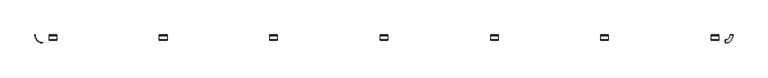
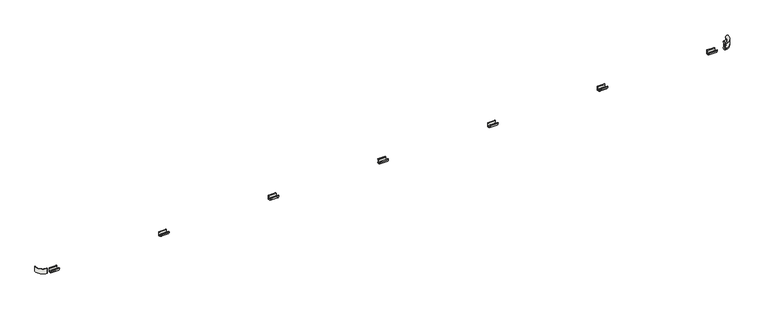
"""IFC4 building model written with IfcOpenShell, lengths in millimetres: covering geometry, Construction_Railing_SPM_Starline-Anodisee-Decowood : Decowood."""

from ifc_helpers import new_model, si_unit, point, frame, frame_2d, origin, place, context, project, spatial, polyline, circle_curve, ellipse_curve, trimmed, segment, composite_curve, outline, extrude, source, transform, mapped, element, save
from ifc_brep_helpers import plane_surface, cylinder_surface, revolved_surface, advanced_brep


def covering_9951a4d6(model_context):
    return source(origin(), model_context, "Body", "SolidModel", [
        advanced_brep(
        [(5562.5, 0.0, 711.0388007), (5562.5, -1.6924902, 711.0388007), (5562.5, -1.6924902, 680.0573863), (5562.5, 0.0, 680.0573863), (5562.5, 0.0, 675.0589555), (5562.5, -4.6960308, 675.0589555), (5562.5, -53.704315, 715.3021276), (5562.5, -51.003274, 720.0337391), (5562.5, -48.3728597, 720.0337391), (5562.5, -11.4596372, 681.5800945), (5562.5, -5.6906152, 686.5206011), (5562.5, -5.6906152, 712.273279), (5562.5, -1.927393, 716.0365012), (5562.5, 0.0, 716.0365012), (5637.5, 0.0, 711.0388007), (5637.5, 0.0, 716.0365012), (5637.5, -1.927393, 716.0365012), (5637.5, -5.6906152, 712.273279), (5637.5, -5.6906152, 686.5206011), (5637.5, -11.4596372, 681.5800945), (5637.5, -48.3728597, 720.0337391), (5637.5, -51.003274, 720.0337391), (5637.5, -53.704315, 715.3021276), (5637.5, -4.6960308, 675.059214), (5637.5, 0.0, 675.0589555), (5637.5, 0.0, 680.0573863), (5637.5, -1.6924902, 680.0573863), (5637.5, -1.6924902, 711.0388007)],
        [
            (0, 1),
            (1, 2),
            (2, 3),
            (3, 4),
            (4, 5),
            (5, 6, circle_curve(frame((5562.5, -4.6960308, 725.0220975), z_axis=(-1.0, 0.0, 0.0), x_axis=(0.0, 0.0, 1.0)), 49.9628835)),
            (6, 7, circle_curve(frame((5562.5, -65.1640589, 724.9806745), z_axis=(1.0, 0.0, 0.0), x_axis=(0.0, 0.0, 1.0)), 15.0)),
            (7, 8),
            (8, 9, circle_curve(frame((5562.5, -4.6988472, 725.0141293), z_axis=(1.0, 0.0, 0.0), x_axis=(0.0, 0.0, 1.0)), 43.957066)),
            (9, 10, circle_curve(frame((5562.5, -10.6906152, 686.5206011), z_axis=(1.0, 0.0, 0.0), x_axis=(0.0, 0.0, 1.0)), 5.0)),
            (10, 11),
            (11, 12, circle_curve(frame((5562.5, -1.927393, 712.273279), z_axis=(-1.0, 0.0, 0.0), x_axis=(0.0, 0.0, 1.0)), 3.7632222)),
            (12, 13),
            (13, 0),
            (14, 15),
            (15, 16),
            (16, 17, circle_curve(frame((5637.5, -1.927393, 712.273279), z_axis=(1.0, 0.0, 0.0), x_axis=(0.0, 0.0, 1.0)), 3.7632222)),
            (17, 18),
            (18, 19, circle_curve(frame((5637.5, -10.6906152, 686.5206011), z_axis=(-1.0, 0.0, 0.0), x_axis=(0.0, 0.0, 1.0)), 5.0)),
            (19, 20, circle_curve(frame((5637.5, -4.6988472, 725.0141293), z_axis=(-1.0, 0.0, 0.0), x_axis=(0.0, 0.0, 1.0)), 43.957066)),
            (20, 21),
            (21, 22, circle_curve(frame((5637.5, -65.1640589, 724.9806745), z_axis=(-1.0, 0.0, 0.0), x_axis=(0.0, 0.0, 1.0)), 15.0)),
            (22, 23, circle_curve(frame((5637.5, -4.6960308, 725.0220975), z_axis=(1.0, 0.0, 0.0), x_axis=(0.0, 0.0, 1.0)), 49.9628835)),
            (23, 24),
            (24, 25),
            (25, 26),
            (26, 27),
            (27, 14),
            (0, 14),
            (27, 1),
            (26, 2),
            (25, 3),
            (24, 4),
            (23, 5),
            (22, 6),
            (21, 7),
            (20, 8),
            (19, 9),
            (18, 10),
            (17, 11),
            (16, 12),
            (15, 13),
        ],
        [
            plane_surface(frame((5562.5, -1.6924902, 711.0388007), z_axis=(-1.0, 0.0, 0.0), x_axis=(0.0, -1.0, 0.0))),
            plane_surface(frame((5637.5, -1.6924902, 711.0388007), z_axis=(1.0, 0.0, 0.0), x_axis=(0.0, 1.0, 0.0))),
            plane_surface(frame((5562.5, 0.0, 711.0388007), z_axis=(0.0, 0.0, -1.0), x_axis=(1.0, 0.0, 0.0))),
            plane_surface(frame((5562.5, -1.6924902, 711.0388007), z_axis=(0.0, 1.0, 0.0), x_axis=(1.0, 0.0, 0.0))),
            plane_surface(frame((5562.5, -1.6924902, 680.0573863), z_axis=(0.0, 0.0, 1.0), x_axis=(1.0, 0.0, 0.0))),
            plane_surface(frame((5562.5, 0.0, 680.0573863), z_axis=(0.0, 1.0, 0.0), x_axis=(1.0, 0.0, 0.0))),
            plane_surface(frame((5562.5, 0.0, 675.0589555), z_axis=(0.0, 0.0, -1.0), x_axis=(1.0, 0.0, 0.0))),
            cylinder_surface(frame((5637.5, -4.6960308, 725.0220975), z_axis=(-1.0, 0.0, 0.0), x_axis=(0.0, 0.0, 1.0)), 49.9628835),
            revolved_surface(polyline([(5637.5, -65.1640589, 739.9806745), (5562.5, -65.1640589, 739.9806745)]), (5637.5, -65.1640589, 724.9806745), (1.0, 0.0, 0.0)),
            plane_surface(frame((5562.5, -51.003274, 720.0337391), z_axis=(0.0, 0.0, 1.0), x_axis=(1.0, 0.0, 0.0))),
            revolved_surface(polyline([(5637.5, -4.6988472, 768.9711953000001), (5562.5, -4.6988472, 768.9711953000001)]), (5637.5, -4.6988472, 725.0141293), (1.0, 0.0, 0.0)),
            revolved_surface(polyline([(5637.5, -10.6906152, 691.5206011), (5562.5, -10.6906152, 691.5206011)]), (5637.5, -10.6906152, 686.5206011), (1.0, 0.0, 0.0)),
            plane_surface(frame((5562.5, -5.6906152, 686.5206011), z_axis=(0.0, -1.0, 0.0), x_axis=(1.0, 0.0, 0.0))),
            cylinder_surface(frame((5637.5, -1.927393, 712.273279), z_axis=(-1.0, 0.0, 0.0), x_axis=(0.0, 0.0, 1.0)), 3.7632222),
            plane_surface(frame((5562.5, -1.927393, 716.0365012), z_axis=(0.0, 0.0, 1.0), x_axis=(1.0, 0.0, 0.0))),
            plane_surface(frame((5562.5, 0.0, 716.0365012), z_axis=(0.0, 1.0, 0.0), x_axis=(1.0, 0.0, 0.0))),
        ],
        [
            (0, [[1, 2, 3, 4, 5, 6, 7, 8, 9, 10, 11, 12, 13, 14]]),
            (1, [[15, 16, 17, 18, 19, 20, 21, 22, 23, 24, 25, 26, 27, 28]]),
            (2, [[-1, 29, -28, 30]]),
            (3, [[-2, -30, -27, 31]]),
            (4, [[-3, -31, -26, 32]]),
            (5, [[-4, -32, -25, 33]]),
            (6, [[-5, -33, -24, 34]]),
            (7, [[-6, -34, -23, 35]]),
            (8, [[-7, -35, -22, 36]]),
            (9, [[-8, -36, -21, 37]]),
            (10, [[-9, -37, -20, 38]]),
            (11, [[-10, -38, -19, 39]]),
            (12, [[-11, -39, -18, 40]]),
            (13, [[-12, -40, -17, 41]]),
            (14, [[-13, -41, -16, 42]]),
            (15, [[-14, -42, -15, -29]]),
        ],
    ),
        advanced_brep(
        [(4462.5, 0.0, 711.0388007), (4462.5, -1.6924902, 711.0388007), (4462.5, -1.6924902, 680.0573863), (4462.5, 0.0, 680.0573863), (4462.5, 0.0, 675.0589555), (4462.5, -4.6960308, 675.0589555), (4462.5, -53.704315, 715.3021276), (4462.5, -51.003274, 720.0337391), (4462.5, -48.3728597, 720.0337391), (4462.5, -11.4596372, 681.5800945), (4462.5, -5.6906152, 686.5206011), (4462.5, -5.6906152, 712.273279), (4462.5, -1.927393, 716.0365012), (4462.5, 0.0, 716.0365012), (4537.5, 0.0, 711.0388007), (4537.5, 0.0, 716.0365012), (4537.5, -1.927393, 716.0365012), (4537.5, -5.6906152, 712.273279), (4537.5, -5.6906152, 686.5206011), (4537.5, -11.4596372, 681.5800945), (4537.5, -48.3728597, 720.0337391), (4537.5, -51.003274, 720.0337391), (4537.5, -53.704315, 715.3021276), (4537.5, -4.6960308, 675.059214), (4537.5, 0.0, 675.0589555), (4537.5, 0.0, 680.0573863), (4537.5, -1.6924902, 680.0573863), (4537.5, -1.6924902, 711.0388007)],
        [
            (0, 1),
            (1, 2),
            (2, 3),
            (3, 4),
            (4, 5),
            (5, 6, circle_curve(frame((4462.5, -4.6960308, 725.0220975), z_axis=(-1.0, 0.0, 0.0), x_axis=(0.0, 0.0, 1.0)), 49.9628835)),
            (6, 7, circle_curve(frame((4462.5, -65.1640589, 724.9806745), z_axis=(1.0, 0.0, 0.0), x_axis=(0.0, 0.0, 1.0)), 15.0)),
            (7, 8),
            (8, 9, circle_curve(frame((4462.5, -4.6988472, 725.0141293), z_axis=(1.0, 0.0, 0.0), x_axis=(0.0, 0.0, 1.0)), 43.957066)),
            (9, 10, circle_curve(frame((4462.5, -10.6906152, 686.5206011), z_axis=(1.0, 0.0, 0.0), x_axis=(0.0, 0.0, 1.0)), 5.0)),
            (10, 11),
            (11, 12, circle_curve(frame((4462.5, -1.927393, 712.273279), z_axis=(-1.0, 0.0, 0.0), x_axis=(0.0, 0.0, 1.0)), 3.7632222)),
            (12, 13),
            (13, 0),
            (14, 15),
            (15, 16),
            (16, 17, circle_curve(frame((4537.5, -1.927393, 712.273279), z_axis=(1.0, 0.0, 0.0), x_axis=(0.0, 0.0, 1.0)), 3.7632222)),
            (17, 18),
            (18, 19, circle_curve(frame((4537.5, -10.6906152, 686.5206011), z_axis=(-1.0, 0.0, 0.0), x_axis=(0.0, 0.0, 1.0)), 5.0)),
            (19, 20, circle_curve(frame((4537.5, -4.6988472, 725.0141293), z_axis=(-1.0, 0.0, 0.0), x_axis=(0.0, 0.0, 1.0)), 43.957066)),
            (20, 21),
            (21, 22, circle_curve(frame((4537.5, -65.1640589, 724.9806745), z_axis=(-1.0, 0.0, 0.0), x_axis=(0.0, 0.0, 1.0)), 15.0)),
            (22, 23, circle_curve(frame((4537.5, -4.6960308, 725.0220975), z_axis=(1.0, 0.0, 0.0), x_axis=(0.0, 0.0, 1.0)), 49.9628835)),
            (23, 24),
            (24, 25),
            (25, 26),
            (26, 27),
            (27, 14),
            (0, 14),
            (27, 1),
            (26, 2),
            (25, 3),
            (24, 4),
            (23, 5),
            (22, 6),
            (21, 7),
            (20, 8),
            (19, 9),
            (18, 10),
            (17, 11),
            (16, 12),
            (15, 13),
        ],
        [
            plane_surface(frame((4462.5, -1.6924902, 711.0388007), z_axis=(-1.0, 0.0, 0.0), x_axis=(0.0, -1.0, 0.0))),
            plane_surface(frame((4537.5, -1.6924902, 711.0388007), z_axis=(1.0, 0.0, 0.0), x_axis=(0.0, 1.0, 0.0))),
            plane_surface(frame((4462.5, 0.0, 711.0388007), z_axis=(0.0, 0.0, -1.0), x_axis=(1.0, 0.0, 0.0))),
            plane_surface(frame((4462.5, -1.6924902, 711.0388007), z_axis=(0.0, 1.0, 0.0), x_axis=(1.0, 0.0, 0.0))),
            plane_surface(frame((4462.5, -1.6924902, 680.0573863), z_axis=(0.0, 0.0, 1.0), x_axis=(1.0, 0.0, 0.0))),
            plane_surface(frame((4462.5, 0.0, 680.0573863), z_axis=(0.0, 1.0, 0.0), x_axis=(1.0, 0.0, 0.0))),
            plane_surface(frame((4462.5, 0.0, 675.0589555), z_axis=(0.0, 0.0, -1.0), x_axis=(1.0, 0.0, 0.0))),
            cylinder_surface(frame((4537.5, -4.6960308, 725.0220975), z_axis=(-1.0, 0.0, 0.0), x_axis=(0.0, 0.0, 1.0)), 49.9628835),
            revolved_surface(polyline([(4537.5, -65.1640589, 739.9806745), (4462.5, -65.1640589, 739.9806745)]), (4537.5, -65.1640589, 724.9806745), (1.0, 0.0, 0.0)),
            plane_surface(frame((4462.5, -51.003274, 720.0337391), z_axis=(0.0, 0.0, 1.0), x_axis=(1.0, 0.0, 0.0))),
            revolved_surface(polyline([(4537.5, -4.6988472, 768.9711953000001), (4462.5, -4.6988472, 768.9711953000001)]), (4537.5, -4.6988472, 725.0141293), (1.0, 0.0, 0.0)),
            revolved_surface(polyline([(4537.5, -10.6906152, 691.5206011), (4462.5, -10.6906152, 691.5206011)]), (4537.5, -10.6906152, 686.5206011), (1.0, 0.0, 0.0)),
            plane_surface(frame((4462.5, -5.6906152, 686.5206011), z_axis=(0.0, -1.0, 0.0), x_axis=(1.0, 0.0, 0.0))),
            cylinder_surface(frame((4537.5, -1.927393, 712.273279), z_axis=(-1.0, 0.0, 0.0), x_axis=(0.0, 0.0, 1.0)), 3.7632222),
            plane_surface(frame((4462.5, -1.927393, 716.0365012), z_axis=(0.0, 0.0, 1.0), x_axis=(1.0, 0.0, 0.0))),
            plane_surface(frame((4462.5, 0.0, 716.0365012), z_axis=(0.0, 1.0, 0.0), x_axis=(1.0, 0.0, 0.0))),
        ],
        [
            (0, [[1, 2, 3, 4, 5, 6, 7, 8, 9, 10, 11, 12, 13, 14]]),
            (1, [[15, 16, 17, 18, 19, 20, 21, 22, 23, 24, 25, 26, 27, 28]]),
            (2, [[-1, 29, -28, 30]]),
            (3, [[-2, -30, -27, 31]]),
            (4, [[-3, -31, -26, 32]]),
            (5, [[-4, -32, -25, 33]]),
            (6, [[-5, -33, -24, 34]]),
            (7, [[-6, -34, -23, 35]]),
            (8, [[-7, -35, -22, 36]]),
            (9, [[-8, -36, -21, 37]]),
            (10, [[-9, -37, -20, 38]]),
            (11, [[-10, -38, -19, 39]]),
            (12, [[-11, -39, -18, 40]]),
            (13, [[-12, -40, -17, 41]]),
            (14, [[-13, -41, -16, 42]]),
            (15, [[-14, -42, -15, -29]]),
        ],
    ),
        advanced_brep(
        [(3362.5, 0.0, 711.0388007), (3362.5, -1.6924902, 711.0388007), (3362.5, -1.6924902, 680.0573863), (3362.5, 0.0, 680.0573863), (3362.5, 0.0, 675.0589555), (3362.5, -4.6960308, 675.0589555), (3362.5, -53.704315, 715.3021276), (3362.5, -51.003274, 720.0337391), (3362.5, -48.3728597, 720.0337391), (3362.5, -11.4596372, 681.5800945), (3362.5, -5.6906152, 686.5206011), (3362.5, -5.6906152, 712.273279), (3362.5, -1.927393, 716.0365012), (3362.5, 0.0, 716.0365012), (3437.5, 0.0, 711.0388007), (3437.5, 0.0, 716.0365012), (3437.5, -1.927393, 716.0365012), (3437.5, -5.6906152, 712.273279), (3437.5, -5.6906152, 686.5206011), (3437.5, -11.4596372, 681.5800945), (3437.5, -48.3728597, 720.0337391), (3437.5, -51.003274, 720.0337391), (3437.5, -53.704315, 715.3021276), (3437.5, -4.6960308, 675.059214), (3437.5, 0.0, 675.0589555), (3437.5, 0.0, 680.0573863), (3437.5, -1.6924902, 680.0573863), (3437.5, -1.6924902, 711.0388007)],
        [
            (0, 1),
            (1, 2),
            (2, 3),
            (3, 4),
            (4, 5),
            (5, 6, circle_curve(frame((3362.5, -4.6960308, 725.0220975), z_axis=(-1.0, 0.0, 0.0), x_axis=(0.0, 0.0, 1.0)), 49.9628835)),
            (6, 7, circle_curve(frame((3362.5, -65.1640589, 724.9806745), z_axis=(1.0, 0.0, 0.0), x_axis=(0.0, 0.0, 1.0)), 15.0)),
            (7, 8),
            (8, 9, circle_curve(frame((3362.5, -4.6988472, 725.0141293), z_axis=(1.0, 0.0, 0.0), x_axis=(0.0, 0.0, 1.0)), 43.957066)),
            (9, 10, circle_curve(frame((3362.5, -10.6906152, 686.5206011), z_axis=(1.0, 0.0, 0.0), x_axis=(0.0, 0.0, 1.0)), 5.0)),
            (10, 11),
            (11, 12, circle_curve(frame((3362.5, -1.927393, 712.273279), z_axis=(-1.0, 0.0, 0.0), x_axis=(0.0, 0.0, 1.0)), 3.7632222)),
            (12, 13),
            (13, 0),
            (14, 15),
            (15, 16),
            (16, 17, circle_curve(frame((3437.5, -1.927393, 712.273279), z_axis=(1.0, 0.0, 0.0), x_axis=(0.0, 0.0, 1.0)), 3.7632222)),
            (17, 18),
            (18, 19, circle_curve(frame((3437.5, -10.6906152, 686.5206011), z_axis=(-1.0, 0.0, 0.0), x_axis=(0.0, 0.0, 1.0)), 5.0)),
            (19, 20, circle_curve(frame((3437.5, -4.6988472, 725.0141293), z_axis=(-1.0, 0.0, 0.0), x_axis=(0.0, 0.0, 1.0)), 43.957066)),
            (20, 21),
            (21, 22, circle_curve(frame((3437.5, -65.1640589, 724.9806745), z_axis=(-1.0, 0.0, 0.0), x_axis=(0.0, 0.0, 1.0)), 15.0)),
            (22, 23, circle_curve(frame((3437.5, -4.6960308, 725.0220975), z_axis=(1.0, 0.0, 0.0), x_axis=(0.0, 0.0, 1.0)), 49.9628835)),
            (23, 24),
            (24, 25),
            (25, 26),
            (26, 27),
            (27, 14),
            (0, 14),
            (27, 1),
            (26, 2),
            (25, 3),
            (24, 4),
            (23, 5),
            (22, 6),
            (21, 7),
            (20, 8),
            (19, 9),
            (18, 10),
            (17, 11),
            (16, 12),
            (15, 13),
        ],
        [
            plane_surface(frame((3362.5, -1.6924902, 711.0388007), z_axis=(-1.0, 0.0, 0.0), x_axis=(0.0, -1.0, 0.0))),
            plane_surface(frame((3437.5, -1.6924902, 711.0388007), z_axis=(1.0, 0.0, 0.0), x_axis=(0.0, 1.0, 0.0))),
            plane_surface(frame((3362.5, 0.0, 711.0388007), z_axis=(0.0, 0.0, -1.0), x_axis=(1.0, 0.0, 0.0))),
            plane_surface(frame((3362.5, -1.6924902, 711.0388007), z_axis=(0.0, 1.0, 0.0), x_axis=(1.0, 0.0, 0.0))),
            plane_surface(frame((3362.5, -1.6924902, 680.0573863), z_axis=(0.0, 0.0, 1.0), x_axis=(1.0, 0.0, 0.0))),
            plane_surface(frame((3362.5, 0.0, 680.0573863), z_axis=(0.0, 1.0, 0.0), x_axis=(1.0, 0.0, 0.0))),
            plane_surface(frame((3362.5, 0.0, 675.0589555), z_axis=(0.0, 0.0, -1.0), x_axis=(1.0, 0.0, 0.0))),
            cylinder_surface(frame((3437.5, -4.6960308, 725.0220975), z_axis=(-1.0, 0.0, 0.0), x_axis=(0.0, 0.0, 1.0)), 49.9628835),
            revolved_surface(polyline([(3437.5, -65.1640589, 739.9806745), (3362.5, -65.1640589, 739.9806745)]), (3437.5, -65.1640589, 724.9806745), (1.0, 0.0, 0.0)),
            plane_surface(frame((3362.5, -51.003274, 720.0337391), z_axis=(0.0, 0.0, 1.0), x_axis=(1.0, 0.0, 0.0))),
            revolved_surface(polyline([(3437.5, -4.6988472, 768.9711953000001), (3362.5, -4.6988472, 768.9711953000001)]), (3437.5, -4.6988472, 725.0141293), (1.0, 0.0, 0.0)),
            revolved_surface(polyline([(3437.5, -10.6906152, 691.5206011), (3362.5, -10.6906152, 691.5206011)]), (3437.5, -10.6906152, 686.5206011), (1.0, 0.0, 0.0)),
            plane_surface(frame((3362.5, -5.6906152, 686.5206011), z_axis=(0.0, -1.0, 0.0), x_axis=(1.0, 0.0, 0.0))),
            cylinder_surface(frame((3437.5, -1.927393, 712.273279), z_axis=(-1.0, 0.0, 0.0), x_axis=(0.0, 0.0, 1.0)), 3.7632222),
            plane_surface(frame((3362.5, -1.927393, 716.0365012), z_axis=(0.0, 0.0, 1.0), x_axis=(1.0, 0.0, 0.0))),
            plane_surface(frame((3362.5, 0.0, 716.0365012), z_axis=(0.0, 1.0, 0.0), x_axis=(1.0, 0.0, 0.0))),
        ],
        [
            (0, [[1, 2, 3, 4, 5, 6, 7, 8, 9, 10, 11, 12, 13, 14]]),
            (1, [[15, 16, 17, 18, 19, 20, 21, 22, 23, 24, 25, 26, 27, 28]]),
            (2, [[-1, 29, -28, 30]]),
            (3, [[-2, -30, -27, 31]]),
            (4, [[-3, -31, -26, 32]]),
            (5, [[-4, -32, -25, 33]]),
            (6, [[-5, -33, -24, 34]]),
            (7, [[-6, -34, -23, 35]]),
            (8, [[-7, -35, -22, 36]]),
            (9, [[-8, -36, -21, 37]]),
            (10, [[-9, -37, -20, 38]]),
            (11, [[-10, -38, -19, 39]]),
            (12, [[-11, -39, -18, 40]]),
            (13, [[-12, -40, -17, 41]]),
            (14, [[-13, -41, -16, 42]]),
            (15, [[-14, -42, -15, -29]]),
        ],
    ),
        advanced_brep(
        [(2262.5, 0.0, 711.0388007), (2262.5, -1.6924902, 711.0388007), (2262.5, -1.6924902, 680.0573863), (2262.5, 0.0, 680.0573863), (2262.5, 0.0, 675.0589555), (2262.5, -4.6960308, 675.0589555), (2262.5, -53.704315, 715.3021276), (2262.5, -51.003274, 720.0337391), (2262.5, -48.3728597, 720.0337391), (2262.5, -11.4596372, 681.5800945), (2262.5, -5.6906152, 686.5206011), (2262.5, -5.6906152, 712.273279), (2262.5, -1.927393, 716.0365012), (2262.5, 0.0, 716.0365012), (2337.5, 0.0, 711.0388007), (2337.5, 0.0, 716.0365012), (2337.5, -1.927393, 716.0365012), (2337.5, -5.6906152, 712.273279), (2337.5, -5.6906152, 686.5206011), (2337.5, -11.4596372, 681.5800945), (2337.5, -48.3728597, 720.0337391), (2337.5, -51.003274, 720.0337391), (2337.5, -53.704315, 715.3021276), (2337.5, -4.6960308, 675.059214), (2337.5, 0.0, 675.0589555), (2337.5, 0.0, 680.0573863), (2337.5, -1.6924902, 680.0573863), (2337.5, -1.6924902, 711.0388007)],
        [
            (0, 1),
            (1, 2),
            (2, 3),
            (3, 4),
            (4, 5),
            (5, 6, circle_curve(frame((2262.5, -4.6960308, 725.0220975), z_axis=(-1.0, 0.0, 0.0), x_axis=(0.0, 0.0, 1.0)), 49.9628835)),
            (6, 7, circle_curve(frame((2262.5, -65.1640589, 724.9806745), z_axis=(1.0, 0.0, 0.0), x_axis=(0.0, 0.0, 1.0)), 15.0)),
            (7, 8),
            (8, 9, circle_curve(frame((2262.5, -4.6988472, 725.0141293), z_axis=(1.0, 0.0, 0.0), x_axis=(0.0, 0.0, 1.0)), 43.957066)),
            (9, 10, circle_curve(frame((2262.5, -10.6906152, 686.5206011), z_axis=(1.0, 0.0, 0.0), x_axis=(0.0, 0.0, 1.0)), 5.0)),
            (10, 11),
            (11, 12, circle_curve(frame((2262.5, -1.927393, 712.273279), z_axis=(-1.0, 0.0, 0.0), x_axis=(0.0, 0.0, 1.0)), 3.7632222)),
            (12, 13),
            (13, 0),
            (14, 15),
            (15, 16),
            (16, 17, circle_curve(frame((2337.5, -1.927393, 712.273279), z_axis=(1.0, 0.0, 0.0), x_axis=(0.0, 0.0, 1.0)), 3.7632222)),
            (17, 18),
            (18, 19, circle_curve(frame((2337.5, -10.6906152, 686.5206011), z_axis=(-1.0, 0.0, 0.0), x_axis=(0.0, 0.0, 1.0)), 5.0)),
            (19, 20, circle_curve(frame((2337.5, -4.6988472, 725.0141293), z_axis=(-1.0, 0.0, 0.0), x_axis=(0.0, 0.0, 1.0)), 43.957066)),
            (20, 21),
            (21, 22, circle_curve(frame((2337.5, -65.1640589, 724.9806745), z_axis=(-1.0, 0.0, 0.0), x_axis=(0.0, 0.0, 1.0)), 15.0)),
            (22, 23, circle_curve(frame((2337.5, -4.6960308, 725.0220975), z_axis=(1.0, 0.0, 0.0), x_axis=(0.0, 0.0, 1.0)), 49.9628835)),
            (23, 24),
            (24, 25),
            (25, 26),
            (26, 27),
            (27, 14),
            (0, 14),
            (27, 1),
            (26, 2),
            (25, 3),
            (24, 4),
            (23, 5),
            (22, 6),
            (21, 7),
            (20, 8),
            (19, 9),
            (18, 10),
            (17, 11),
            (16, 12),
            (15, 13),
        ],
        [
            plane_surface(frame((2262.5, -1.6924902, 711.0388007), z_axis=(-1.0, 0.0, 0.0), x_axis=(0.0, -1.0, 0.0))),
            plane_surface(frame((2337.5, -1.6924902, 711.0388007), z_axis=(1.0, 0.0, 0.0), x_axis=(0.0, 1.0, 0.0))),
            plane_surface(frame((2262.5, 0.0, 711.0388007), z_axis=(0.0, 0.0, -1.0), x_axis=(1.0, 0.0, 0.0))),
            plane_surface(frame((2262.5, -1.6924902, 711.0388007), z_axis=(0.0, 1.0, 0.0), x_axis=(1.0, 0.0, 0.0))),
            plane_surface(frame((2262.5, -1.6924902, 680.0573863), z_axis=(0.0, 0.0, 1.0), x_axis=(1.0, 0.0, 0.0))),
            plane_surface(frame((2262.5, 0.0, 680.0573863), z_axis=(0.0, 1.0, 0.0), x_axis=(1.0, 0.0, 0.0))),
            plane_surface(frame((2262.5, 0.0, 675.0589555), z_axis=(0.0, 0.0, -1.0), x_axis=(1.0, 0.0, 0.0))),
            cylinder_surface(frame((2337.5, -4.6960308, 725.0220975), z_axis=(-1.0, 0.0, 0.0), x_axis=(0.0, 0.0, 1.0)), 49.9628835),
            revolved_surface(polyline([(2337.5, -65.1640589, 739.9806745), (2262.5, -65.1640589, 739.9806745)]), (2337.5, -65.1640589, 724.9806745), (1.0, 0.0, 0.0)),
            plane_surface(frame((2262.5, -51.003274, 720.0337391), z_axis=(0.0, 0.0, 1.0), x_axis=(1.0, 0.0, 0.0))),
            revolved_surface(polyline([(2337.5, -4.6988472, 768.9711953000001), (2262.5, -4.6988472, 768.9711953000001)]), (2337.5, -4.6988472, 725.0141293), (1.0, 0.0, 0.0)),
            revolved_surface(polyline([(2337.5, -10.6906152, 691.5206011), (2262.5, -10.6906152, 691.5206011)]), (2337.5, -10.6906152, 686.5206011), (1.0, 0.0, 0.0)),
            plane_surface(frame((2262.5, -5.6906152, 686.5206011), z_axis=(0.0, -1.0, 0.0), x_axis=(1.0, 0.0, 0.0))),
            cylinder_surface(frame((2337.5, -1.927393, 712.273279), z_axis=(-1.0, 0.0, 0.0), x_axis=(0.0, 0.0, 1.0)), 3.7632222),
            plane_surface(frame((2262.5, -1.927393, 716.0365012), z_axis=(0.0, 0.0, 1.0), x_axis=(1.0, 0.0, 0.0))),
            plane_surface(frame((2262.5, 0.0, 716.0365012), z_axis=(0.0, 1.0, 0.0), x_axis=(1.0, 0.0, 0.0))),
        ],
        [
            (0, [[1, 2, 3, 4, 5, 6, 7, 8, 9, 10, 11, 12, 13, 14]]),
            (1, [[15, 16, 17, 18, 19, 20, 21, 22, 23, 24, 25, 26, 27, 28]]),
            (2, [[-1, 29, -28, 30]]),
            (3, [[-2, -30, -27, 31]]),
            (4, [[-3, -31, -26, 32]]),
            (5, [[-4, -32, -25, 33]]),
            (6, [[-5, -33, -24, 34]]),
            (7, [[-6, -34, -23, 35]]),
            (8, [[-7, -35, -22, 36]]),
            (9, [[-8, -36, -21, 37]]),
            (10, [[-9, -37, -20, 38]]),
            (11, [[-10, -38, -19, 39]]),
            (12, [[-11, -39, -18, 40]]),
            (13, [[-12, -40, -17, 41]]),
            (14, [[-13, -41, -16, 42]]),
            (15, [[-14, -42, -15, -29]]),
        ],
    ),
        advanced_brep(
        [(1162.5, 0.0, 711.0388007), (1162.5, -1.6924902, 711.0388007), (1162.5, -1.6924902, 680.0573863), (1162.5, 0.0, 680.0573863), (1162.5, 0.0, 675.0589555), (1162.5, -4.6960308, 675.0589555), (1162.5, -53.704315, 715.3021276), (1162.5, -51.003274, 720.0337391), (1162.5, -48.3728597, 720.0337391), (1162.5, -11.4596372, 681.5800945), (1162.5, -5.6906152, 686.5206011), (1162.5, -5.6906152, 712.273279), (1162.5, -1.927393, 716.0365012), (1162.5, 0.0, 716.0365012), (1237.5, 0.0, 711.0388007), (1237.5, 0.0, 716.0365012), (1237.5, -1.927393, 716.0365012), (1237.5, -5.6906152, 712.273279), (1237.5, -5.6906152, 686.5206011), (1237.5, -11.4596372, 681.5800945), (1237.5, -48.3728597, 720.0337391), (1237.5, -51.003274, 720.0337391), (1237.5, -53.704315, 715.3021276), (1237.5, -4.6960308, 675.059214), (1237.5, 0.0, 675.0589555), (1237.5, 0.0, 680.0573863), (1237.5, -1.6924902, 680.0573863), (1237.5, -1.6924902, 711.0388007)],
        [
            (0, 1),
            (1, 2),
            (2, 3),
            (3, 4),
            (4, 5),
            (5, 6, circle_curve(frame((1162.5, -4.6960308, 725.0220975), z_axis=(-1.0, 0.0, 0.0), x_axis=(0.0, 0.0, 1.0)), 49.9628835)),
            (6, 7, circle_curve(frame((1162.5, -65.1640589, 724.9806745), z_axis=(1.0, 0.0, 0.0), x_axis=(0.0, 0.0, 1.0)), 15.0)),
            (7, 8),
            (8, 9, circle_curve(frame((1162.5, -4.6988472, 725.0141293), z_axis=(1.0, 0.0, 0.0), x_axis=(0.0, 0.0, 1.0)), 43.957066)),
            (9, 10, circle_curve(frame((1162.5, -10.6906152, 686.5206011), z_axis=(1.0, 0.0, 0.0), x_axis=(0.0, 0.0, 1.0)), 5.0)),
            (10, 11),
            (11, 12, circle_curve(frame((1162.5, -1.927393, 712.273279), z_axis=(-1.0, 0.0, 0.0), x_axis=(0.0, 0.0, 1.0)), 3.7632222)),
            (12, 13),
            (13, 0),
            (14, 15),
            (15, 16),
            (16, 17, circle_curve(frame((1237.5, -1.927393, 712.273279), z_axis=(1.0, 0.0, 0.0), x_axis=(0.0, 0.0, 1.0)), 3.7632222)),
            (17, 18),
            (18, 19, circle_curve(frame((1237.5, -10.6906152, 686.5206011), z_axis=(-1.0, 0.0, 0.0), x_axis=(0.0, 0.0, 1.0)), 5.0)),
            (19, 20, circle_curve(frame((1237.5, -4.6988472, 725.0141293), z_axis=(-1.0, 0.0, 0.0), x_axis=(0.0, 0.0, 1.0)), 43.957066)),
            (20, 21),
            (21, 22, circle_curve(frame((1237.5, -65.1640589, 724.9806745), z_axis=(-1.0, 0.0, 0.0), x_axis=(0.0, 0.0, 1.0)), 15.0)),
            (22, 23, circle_curve(frame((1237.5, -4.6960308, 725.0220975), z_axis=(1.0, 0.0, 0.0), x_axis=(0.0, 0.0, 1.0)), 49.9628835)),
            (23, 24),
            (24, 25),
            (25, 26),
            (26, 27),
            (27, 14),
            (0, 14),
            (27, 1),
            (26, 2),
            (25, 3),
            (24, 4),
            (23, 5),
            (22, 6),
            (21, 7),
            (20, 8),
            (19, 9),
            (18, 10),
            (17, 11),
            (16, 12),
            (15, 13),
        ],
        [
            plane_surface(frame((1162.5, -1.6924902, 711.0388007), z_axis=(-1.0, 0.0, 0.0), x_axis=(0.0, -1.0, 0.0))),
            plane_surface(frame((1237.5, -1.6924902, 711.0388007), z_axis=(1.0, 0.0, 0.0), x_axis=(0.0, 1.0, 0.0))),
            plane_surface(frame((1162.5, 0.0, 711.0388007), z_axis=(0.0, 0.0, -1.0), x_axis=(1.0, 0.0, 0.0))),
            plane_surface(frame((1162.5, -1.6924902, 711.0388007), z_axis=(0.0, 1.0, 0.0), x_axis=(1.0, 0.0, 0.0))),
            plane_surface(frame((1162.5, -1.6924902, 680.0573863), z_axis=(0.0, 0.0, 1.0), x_axis=(1.0, 0.0, 0.0))),
            plane_surface(frame((1162.5, 0.0, 680.0573863), z_axis=(0.0, 1.0, 0.0), x_axis=(1.0, 0.0, 0.0))),
            plane_surface(frame((1162.5, 0.0, 675.0589555), z_axis=(0.0, 0.0, -1.0), x_axis=(1.0, 0.0, 0.0))),
            cylinder_surface(frame((1237.5, -4.6960308, 725.0220975), z_axis=(-1.0, 0.0, 0.0), x_axis=(0.0, 0.0, 1.0)), 49.9628835),
            revolved_surface(polyline([(1237.5, -65.1640589, 739.9806745), (1162.5, -65.1640589, 739.9806745)]), (1237.5, -65.1640589, 724.9806745), (1.0, 0.0, 0.0)),
            plane_surface(frame((1162.5, -51.003274, 720.0337391), z_axis=(0.0, 0.0, 1.0), x_axis=(1.0, 0.0, 0.0))),
            revolved_surface(polyline([(1237.5, -4.6988472, 768.9711953000001), (1162.5, -4.6988472, 768.9711953000001)]), (1237.5, -4.6988472, 725.0141293), (1.0, 0.0, 0.0)),
            revolved_surface(polyline([(1237.5, -10.6906152, 691.5206011), (1162.5, -10.6906152, 691.5206011)]), (1237.5, -10.6906152, 686.5206011), (1.0, 0.0, 0.0)),
            plane_surface(frame((1162.5, -5.6906152, 686.5206011), z_axis=(0.0, -1.0, 0.0), x_axis=(1.0, 0.0, 0.0))),
            cylinder_surface(frame((1237.5, -1.927393, 712.273279), z_axis=(-1.0, 0.0, 0.0), x_axis=(0.0, 0.0, 1.0)), 3.7632222),
            plane_surface(frame((1162.5, -1.927393, 716.0365012), z_axis=(0.0, 0.0, 1.0), x_axis=(1.0, 0.0, 0.0))),
            plane_surface(frame((1162.5, 0.0, 716.0365012), z_axis=(0.0, 1.0, 0.0), x_axis=(1.0, 0.0, 0.0))),
        ],
        [
            (0, [[1, 2, 3, 4, 5, 6, 7, 8, 9, 10, 11, 12, 13, 14]]),
            (1, [[15, 16, 17, 18, 19, 20, 21, 22, 23, 24, 25, 26, 27, 28]]),
            (2, [[-1, 29, -28, 30]]),
            (3, [[-2, -30, -27, 31]]),
            (4, [[-3, -31, -26, 32]]),
            (5, [[-4, -32, -25, 33]]),
            (6, [[-5, -33, -24, 34]]),
            (7, [[-6, -34, -23, 35]]),
            (8, [[-7, -35, -22, 36]]),
            (9, [[-8, -36, -21, 37]]),
            (10, [[-9, -37, -20, 38]]),
            (11, [[-10, -38, -19, 39]]),
            (12, [[-11, -39, -18, 40]]),
            (13, [[-12, -40, -17, 41]]),
            (14, [[-13, -41, -16, 42]]),
            (15, [[-14, -42, -15, -29]]),
        ],
    ),
        advanced_brep(
        [(6662.5, 0.0, 711.0388007), (6662.5, -1.6924902, 711.0388007), (6662.5, -1.6924902, 680.0573863), (6662.5, 0.0, 680.0573863), (6662.5, 0.0, 675.0589555), (6662.5, -4.6960308, 675.0589555), (6662.5, -53.704315, 715.3021276), (6662.5, -51.003274, 720.0337391), (6662.5, -48.3728597, 720.0337391), (6662.5, -11.4596372, 681.5800945), (6662.5, -5.6906152, 686.5206011), (6662.5, -5.6906152, 712.273279), (6662.5, -1.927393, 716.0365012), (6662.5, 0.0, 716.0365012), (6737.5, 0.0, 711.0388007), (6737.5, 0.0, 716.0365012), (6737.5, -1.927393, 716.0365012), (6737.5, -5.6906152, 712.273279), (6737.5, -5.6906152, 686.5206011), (6737.5, -11.4596372, 681.5800945), (6737.5, -48.3728597, 720.0337391), (6737.5, -51.003274, 720.0337391), (6737.5, -53.704315, 715.3021276), (6737.5, -4.6960308, 675.059214), (6737.5, 0.0, 675.0589555), (6737.5, 0.0, 680.0573863), (6737.5, -1.6924902, 680.0573863), (6737.5, -1.6924902, 711.0388007)],
        [
            (0, 1),
            (1, 2),
            (2, 3),
            (3, 4),
            (4, 5),
            (5, 6, circle_curve(frame((6662.5, -4.6960308, 725.0220975), z_axis=(-1.0, 0.0, 0.0), x_axis=(0.0, 0.0, 1.0)), 49.9628835)),
            (6, 7, circle_curve(frame((6662.5, -65.1640589, 724.9806745), z_axis=(1.0, 0.0, 0.0), x_axis=(0.0, 0.0, 1.0)), 15.0)),
            (7, 8),
            (8, 9, circle_curve(frame((6662.5, -4.6988472, 725.0141293), z_axis=(1.0, 0.0, 0.0), x_axis=(0.0, 0.0, 1.0)), 43.957066)),
            (9, 10, circle_curve(frame((6662.5, -10.6906152, 686.5206011), z_axis=(1.0, 0.0, 0.0), x_axis=(0.0, 0.0, 1.0)), 5.0)),
            (10, 11),
            (11, 12, circle_curve(frame((6662.5, -1.927393, 712.273279), z_axis=(-1.0, 0.0, 0.0), x_axis=(0.0, 0.0, 1.0)), 3.7632222)),
            (12, 13),
            (13, 0),
            (14, 15),
            (15, 16),
            (16, 17, circle_curve(frame((6737.5, -1.927393, 712.273279), z_axis=(1.0, 0.0, 0.0), x_axis=(0.0, 0.0, 1.0)), 3.7632222)),
            (17, 18),
            (18, 19, circle_curve(frame((6737.5, -10.6906152, 686.5206011), z_axis=(-1.0, 0.0, 0.0), x_axis=(0.0, 0.0, 1.0)), 5.0)),
            (19, 20, circle_curve(frame((6737.5, -4.6988472, 725.0141293), z_axis=(-1.0, 0.0, 0.0), x_axis=(0.0, 0.0, 1.0)), 43.957066)),
            (20, 21),
            (21, 22, circle_curve(frame((6737.5, -65.1640589, 724.9806745), z_axis=(-1.0, 0.0, 0.0), x_axis=(0.0, 0.0, 1.0)), 15.0)),
            (22, 23, circle_curve(frame((6737.5, -4.6960308, 725.0220975), z_axis=(1.0, 0.0, 0.0), x_axis=(0.0, 0.0, 1.0)), 49.9628835)),
            (23, 24),
            (24, 25),
            (25, 26),
            (26, 27),
            (27, 14),
            (0, 14),
            (27, 1),
            (26, 2),
            (25, 3),
            (24, 4),
            (23, 5),
            (22, 6),
            (21, 7),
            (20, 8),
            (19, 9),
            (18, 10),
            (17, 11),
            (16, 12),
            (15, 13),
        ],
        [
            plane_surface(frame((6662.5, -1.6924902, 711.0388007), z_axis=(-1.0, 0.0, 0.0), x_axis=(0.0, -1.0, 0.0))),
            plane_surface(frame((6737.5, -1.6924902, 711.0388007), z_axis=(1.0, 0.0, 0.0), x_axis=(0.0, 1.0, 0.0))),
            plane_surface(frame((6662.5, 0.0, 711.0388007), z_axis=(0.0, 0.0, -1.0), x_axis=(1.0, 0.0, 0.0))),
            plane_surface(frame((6662.5, -1.6924902, 711.0388007), z_axis=(0.0, 1.0, 0.0), x_axis=(1.0, 0.0, 0.0))),
            plane_surface(frame((6662.5, -1.6924902, 680.0573863), z_axis=(0.0, 0.0, 1.0), x_axis=(1.0, 0.0, 0.0))),
            plane_surface(frame((6662.5, 0.0, 680.0573863), z_axis=(0.0, 1.0, 0.0), x_axis=(1.0, 0.0, 0.0))),
            plane_surface(frame((6662.5, 0.0, 675.0589555), z_axis=(0.0, 0.0, -1.0), x_axis=(1.0, 0.0, 0.0))),
            cylinder_surface(frame((6737.5, -4.6960308, 725.0220975), z_axis=(-1.0, 0.0, 0.0), x_axis=(0.0, 0.0, 1.0)), 49.9628835),
            revolved_surface(polyline([(6737.5, -65.1640589, 739.9806745), (6662.5, -65.1640589, 739.9806745)]), (6737.5, -65.1640589, 724.9806745), (1.0, 0.0, 0.0)),
            plane_surface(frame((6662.5, -51.003274, 720.0337391), z_axis=(0.0, 0.0, 1.0), x_axis=(1.0, 0.0, 0.0))),
            revolved_surface(polyline([(6737.5, -4.6988472, 768.9711953000001), (6662.5, -4.6988472, 768.9711953000001)]), (6737.5, -4.6988472, 725.0141293), (1.0, 0.0, 0.0)),
            revolved_surface(polyline([(6737.5, -10.6906152, 691.5206011), (6662.5, -10.6906152, 691.5206011)]), (6737.5, -10.6906152, 686.5206011), (1.0, 0.0, 0.0)),
            plane_surface(frame((6662.5, -5.6906152, 686.5206011), z_axis=(0.0, -1.0, 0.0), x_axis=(1.0, 0.0, 0.0))),
            cylinder_surface(frame((6737.5, -1.927393, 712.273279), z_axis=(-1.0, 0.0, 0.0), x_axis=(0.0, 0.0, 1.0)), 3.7632222),
            plane_surface(frame((6662.5, -1.927393, 716.0365012), z_axis=(0.0, 0.0, 1.0), x_axis=(1.0, 0.0, 0.0))),
            plane_surface(frame((6662.5, 0.0, 716.0365012), z_axis=(0.0, 1.0, 0.0), x_axis=(1.0, 0.0, 0.0))),
        ],
        [
            (0, [[1, 2, 3, 4, 5, 6, 7, 8, 9, 10, 11, 12, 13, 14]]),
            (1, [[15, 16, 17, 18, 19, 20, 21, 22, 23, 24, 25, 26, 27, 28]]),
            (2, [[-1, 29, -28, 30]]),
            (3, [[-2, -30, -27, 31]]),
            (4, [[-3, -31, -26, 32]]),
            (5, [[-4, -32, -25, 33]]),
            (6, [[-5, -33, -24, 34]]),
            (7, [[-6, -34, -23, 35]]),
            (8, [[-7, -35, -22, 36]]),
            (9, [[-8, -36, -21, 37]]),
            (10, [[-9, -37, -20, 38]]),
            (11, [[-10, -38, -19, 39]]),
            (12, [[-11, -39, -18, 40]]),
            (13, [[-12, -40, -17, 41]]),
            (14, [[-13, -41, -16, 42]]),
            (15, [[-14, -42, -15, -29]]),
        ],
    ),
        advanced_brep(
        [(62.5, 0.0, 711.0388007), (62.5, -1.6924902, 711.0388007), (62.5, -1.6924902, 680.0573863), (62.5, 0.0, 680.0573863), (62.5, 0.0, 675.0589555), (62.5, -4.6960308, 675.0589555), (62.5, -53.704315, 715.3021276), (62.5, -51.003274, 720.0337391), (62.5, -48.3728597, 720.0337391), (62.5, -11.4596372, 681.5800945), (62.5, -5.6906152, 686.5206011), (62.5, -5.6906152, 712.273279), (62.5, -1.927393, 716.0365012), (62.5, 0.0, 716.0365012), (137.5, 0.0, 711.0388007), (137.5, 0.0, 716.0365012), (137.5, -1.927393, 716.0365012), (137.5, -5.6906152, 712.273279), (137.5, -5.6906152, 686.5206011), (137.5, -11.4596372, 681.5800945), (137.5, -48.3728597, 720.0337391), (137.5, -51.003274, 720.0337391), (137.5, -53.704315, 715.3021276), (137.5, -4.6960308, 675.059214), (137.5, 0.0, 675.0589555), (137.5, 0.0, 680.0573863), (137.5, -1.6924902, 680.0573863), (137.5, -1.6924902, 711.0388007)],
        [
            (0, 1),
            (1, 2),
            (2, 3),
            (3, 4),
            (4, 5),
            (5, 6, circle_curve(frame((62.5, -4.6960308, 725.0220975), z_axis=(-1.0, 0.0, 0.0), x_axis=(0.0, 0.0, 1.0)), 49.9628835)),
            (6, 7, circle_curve(frame((62.5, -65.1640589, 724.9806745), z_axis=(1.0, 0.0, 0.0), x_axis=(0.0, 0.0, 1.0)), 15.0)),
            (7, 8),
            (8, 9, circle_curve(frame((62.5, -4.6988472, 725.0141293), z_axis=(1.0, 0.0, 0.0), x_axis=(0.0, 0.0, 1.0)), 43.957066)),
            (9, 10, circle_curve(frame((62.5, -10.6906152, 686.5206011), z_axis=(1.0, 0.0, 0.0), x_axis=(0.0, 0.0, 1.0)), 5.0)),
            (10, 11),
            (11, 12, circle_curve(frame((62.5, -1.927393, 712.273279), z_axis=(-1.0, 0.0, 0.0), x_axis=(0.0, 0.0, 1.0)), 3.7632222)),
            (12, 13),
            (13, 0),
            (14, 15),
            (15, 16),
            (16, 17, circle_curve(frame((137.5, -1.927393, 712.273279), z_axis=(1.0, 0.0, 0.0), x_axis=(0.0, 0.0, 1.0)), 3.7632222)),
            (17, 18),
            (18, 19, circle_curve(frame((137.5, -10.6906152, 686.5206011), z_axis=(-1.0, 0.0, 0.0), x_axis=(0.0, 0.0, 1.0)), 5.0)),
            (19, 20, circle_curve(frame((137.5, -4.6988472, 725.0141293), z_axis=(-1.0, 0.0, 0.0), x_axis=(0.0, 0.0, 1.0)), 43.957066)),
            (20, 21),
            (21, 22, circle_curve(frame((137.5, -65.1640589, 724.9806745), z_axis=(-1.0, 0.0, 0.0), x_axis=(0.0, 0.0, 1.0)), 15.0)),
            (22, 23, circle_curve(frame((137.5, -4.6960308, 725.0220975), z_axis=(1.0, 0.0, 0.0), x_axis=(0.0, 0.0, 1.0)), 49.9628835)),
            (23, 24),
            (24, 25),
            (25, 26),
            (26, 27),
            (27, 14),
            (0, 14),
            (27, 1),
            (26, 2),
            (25, 3),
            (24, 4),
            (23, 5),
            (22, 6),
            (21, 7),
            (20, 8),
            (19, 9),
            (18, 10),
            (17, 11),
            (16, 12),
            (15, 13),
        ],
        [
            plane_surface(frame((62.5, -1.6924902, 711.0388007), z_axis=(-1.0, 0.0, 0.0), x_axis=(0.0, -1.0, 0.0))),
            plane_surface(frame((137.5, -1.6924902, 711.0388007), z_axis=(1.0, 0.0, 0.0), x_axis=(0.0, 1.0, 0.0))),
            plane_surface(frame((62.5, 0.0, 711.0388007), z_axis=(0.0, 0.0, -1.0), x_axis=(1.0, 0.0, 0.0))),
            plane_surface(frame((62.5, -1.6924902, 711.0388007), z_axis=(0.0, 1.0, 0.0), x_axis=(1.0, 0.0, 0.0))),
            plane_surface(frame((62.5, -1.6924902, 680.0573863), z_axis=(0.0, 0.0, 1.0), x_axis=(1.0, 0.0, 0.0))),
            plane_surface(frame((62.5, 0.0, 680.0573863), z_axis=(0.0, 1.0, 0.0), x_axis=(1.0, 0.0, 0.0))),
            plane_surface(frame((62.5, 0.0, 675.0589555), z_axis=(0.0, 0.0, -1.0), x_axis=(1.0, 0.0, 0.0))),
            cylinder_surface(frame((137.5, -4.6960308, 725.0220975), z_axis=(-1.0, 0.0, 0.0), x_axis=(0.0, 0.0, 1.0)), 49.9628835),
            revolved_surface(polyline([(137.5, -65.1640589, 739.9806745), (62.5, -65.1640589, 739.9806745)]), (137.5, -65.1640589, 724.9806745), (1.0, 0.0, 0.0)),
            plane_surface(frame((62.5, -51.003274, 720.0337391), z_axis=(0.0, 0.0, 1.0), x_axis=(1.0, 0.0, 0.0))),
            revolved_surface(polyline([(137.5, -4.6988472, 768.9711953000001), (62.5, -4.6988472, 768.9711953000001)]), (137.5, -4.6988472, 725.0141293), (1.0, 0.0, 0.0)),
            revolved_surface(polyline([(137.5, -10.6906152, 691.5206011), (62.5, -10.6906152, 691.5206011)]), (137.5, -10.6906152, 686.5206011), (1.0, 0.0, 0.0)),
            plane_surface(frame((62.5, -5.6906152, 686.5206011), z_axis=(0.0, -1.0, 0.0), x_axis=(1.0, 0.0, 0.0))),
            cylinder_surface(frame((137.5, -1.927393, 712.273279), z_axis=(-1.0, 0.0, 0.0), x_axis=(0.0, 0.0, 1.0)), 3.7632222),
            plane_surface(frame((62.5, -1.927393, 716.0365012), z_axis=(0.0, 0.0, 1.0), x_axis=(1.0, 0.0, 0.0))),
            plane_surface(frame((62.5, 0.0, 716.0365012), z_axis=(0.0, 1.0, 0.0), x_axis=(1.0, 0.0, 0.0))),
        ],
        [
            (0, [[1, 2, 3, 4, 5, 6, 7, 8, 9, 10, 11, 12, 13, 14]]),
            (1, [[15, 16, 17, 18, 19, 20, 21, 22, 23, 24, 25, 26, 27, 28]]),
            (2, [[-1, 29, -28, 30]]),
            (3, [[-2, -30, -27, 31]]),
            (4, [[-3, -31, -26, 32]]),
            (5, [[-4, -32, -25, 33]]),
            (6, [[-5, -33, -24, 34]]),
            (7, [[-6, -34, -23, 35]]),
            (8, [[-7, -35, -22, 36]]),
            (9, [[-8, -36, -21, 37]]),
            (10, [[-9, -37, -20, 38]]),
            (11, [[-10, -38, -19, 39]]),
            (12, [[-11, -39, -18, 40]]),
            (13, [[-12, -40, -17, 41]]),
            (14, [[-13, -41, -16, 42]]),
            (15, [[-14, -42, -15, -29]]),
        ],
    ),
        extrude(outline(composite_curve([segment(polyline([(6800.0, -79.3173438), (6800.0, -77.7797808), (6801.0, -77.7797808)]), True, "CONTINUOUS"), segment(trimmed(circle_curve(frame_2d((6801.0, -1.0)), 76.7797808), [point((6801.0, -77.7797808))], [point((6877.7797808, -1.0))], True, "CARTESIAN"), True, "CONTINUOUS"), segment(polyline([(6877.7797808, -1.0), (6877.7797808, 0.0), (6879.3173438, 0.0), (6879.3173438, -1.0)]), True, "CONTINUOUS"), segment(trimmed(circle_curve(frame_2d((6801.0, -1.0)), 78.3173438), [point((6879.3173438, -1.0))], [point((6801.0, -79.3173438))], False, "CARTESIAN"), True, "CONTINUOUS"), segment(polyline([(6801.0, -79.3173438), (6800.0, -79.3173438)]), True, "CONTINUOUS")], self_intersect=False)), frame((0.0, 0.0, 730.187687), z_axis=(0.0, 0.0, 1.0), x_axis=(1.0, 0.0, 0.0)), (0.0, 0.0, 1.0), 49.6510297),
        advanced_brep(
        [(6800.0, -52.1949146, 777.1298269), (6800.0, -52.1949146, 732.7970729), (6800.0, -79.0444967, 730.187687), (6800.0, -77.7797808, 730.187687), (6800.0, -77.7797808, 779.8387167), (6800.0, -78.97282, 779.8387167), (6801.0, -78.97282, 779.8387167), (6801.0, -52.1949146, 777.1298269), (6801.0, -77.7797808, 779.8387167), (6877.7797808, -1.0, 779.8387167), (6877.7797808, 0.0, 779.8387167), (6878.97282, 0.0, 779.8387167), (6878.97282, -1.0, 779.8387167), (6801.0, -77.7797808, 730.187687), (6801.0, -79.0444967, 730.187687), (6879.0444967, -1.0, 730.187687), (6879.0444967, 0.0, 730.187687), (6877.7797808, 0.0, 730.187687), (6877.7797808, -1.0, 730.187687), (6801.0, -52.1949146, 732.7970729), (6852.1949146, -1.0, 777.1298269), (6852.1949146, -1.0, 732.7970729), (6852.1949146, 0.0, 777.1298269), (6852.1949146, 0.0, 732.7970729)],
        [
            (0, 1),
            (1, 2, circle_curve(frame((6800.0, -64.9833199, 724.9442146), z_axis=(-1.0, 0.0, 0.0), x_axis=(0.0, 1.0, 0.0)), 15.0070215)),
            (2, 3),
            (3, 4),
            (4, 5),
            (5, 0, circle_curve(frame((6800.0, -64.921376, 785.0331273), z_axis=(-1.0, 0.0, 0.0), x_axis=(0.0, 1.0, 0.0)), 14.9808204)),
            (5, 6),
            (6, 7, circle_curve(frame((6801.0, -64.921376, 785.0331273), z_axis=(-1.0, 0.0, 0.0), x_axis=(0.0, 1.0, 0.0)), 14.9808204)),
            (7, 0),
            (4, 8),
            (8, 9, circle_curve(frame((6801.0, -1.0, 779.8387167), z_axis=(0.0, 0.0, 1.0), x_axis=(0.0, -1.0, 0.0)), 76.7797808)),
            (9, 10),
            (10, 11),
            (11, 12),
            (12, 6, circle_curve(frame((6801.0, -1.0, 779.8387167), z_axis=(0.0, 0.0, -1.0), x_axis=(0.0, -1.0, 0.0)), 77.97282)),
            (3, 13),
            (13, 8),
            (2, 14),
            (14, 15, circle_curve(frame((6801.0, -1.0, 730.187687), z_axis=(0.0, 0.0, 1.0), x_axis=(0.0, -1.0, 0.0)), 78.0444967)),
            (15, 16),
            (16, 17),
            (17, 18),
            (18, 13, circle_curve(frame((6801.0, -1.0, 730.187687), z_axis=(0.0, 0.0, -1.0), x_axis=(0.0, -1.0, 0.0)), 76.7797808)),
            (1, 19),
            (19, 14, circle_curve(frame((6801.0, -64.9833199, 724.9442146), z_axis=(-1.0, 0.0, 0.0), x_axis=(0.0, 1.0, 0.0)), 15.0070215)),
            (7, 19),
            (20, 7, circle_curve(frame((6801.0, -1.0, 777.1298269), z_axis=(0.0, 0.0, -1.0), x_axis=(0.0, -1.0, 0.0)), 51.1949146)),
            (12, 20, circle_curve(frame((6864.921376, -1.0, 785.0331273), z_axis=(0.0, -1.0, 0.0), x_axis=(-1.0, 0.0, 0.0)), 14.9808204)),
            (18, 9),
            (19, 21, circle_curve(frame((6801.0, -1.0, 732.7970729), z_axis=(0.0, 0.0, 1.0), x_axis=(0.0, -1.0, 0.0)), 51.1949146)),
            (21, 15, circle_curve(frame((6864.9833199, -1.0, 724.9442146), z_axis=(0.0, -1.0, 0.0), x_axis=(-1.0, 0.0, 0.0)), 15.0070215)),
            (20, 21),
            (22, 11, circle_curve(frame((6864.921376, 0.0, 785.0331273), z_axis=(0.0, 1.0, 0.0), x_axis=(-1.0, 0.0, 0.0)), 14.9808204)),
            (10, 17),
            (16, 23, circle_curve(frame((6864.9833199, 0.0, 724.9442146), z_axis=(0.0, 1.0, 0.0), x_axis=(-1.0, 0.0, 0.0)), 15.0070215)),
            (23, 22),
            (22, 20),
            (21, 23),
        ],
        [
            plane_surface(frame((6800.0, -50.0, 710.0), z_axis=(-1.0, 0.0, 0.0), x_axis=(0.0, 0.0, 1.0))),
            cylinder_surface(frame((6800.0, -64.921376, 785.0331273), z_axis=(-1.0, 0.0, 0.0), x_axis=(0.0, 1.0, 0.0)), 14.9808204),
            plane_surface(frame((6800.0, -77.7797808, 779.8387167), z_axis=(0.0, 0.0, -1.0), x_axis=(1.0, 0.0, 0.0))),
            plane_surface(frame((6800.0, -77.7797808, 730.187687), z_axis=(0.0, -1.0, 0.0), x_axis=(1.0, 0.0, 0.0))),
            plane_surface(frame((6800.0, -79.0444967, 730.187687), z_axis=(0.0, 0.0, 1.0), x_axis=(1.0, 0.0, 0.0))),
            cylinder_surface(frame((6800.0, -64.9833199, 724.9442146), z_axis=(-1.0, 0.0, 0.0), x_axis=(0.0, 1.0, 0.0)), 15.0070215),
            plane_surface(frame((6800.0, -52.1949146, 777.1298269), z_axis=(0.0, 1.0, 0.0), x_axis=(1.0, 0.0, 0.0))),
            revolved_surface(trimmed(ellipse_curve(frame((6801.0, -64.921376, 785.0331273), z_axis=(-1.0, 0.0, 0.0), x_axis=(0.0, 1.0, 0.0)), 14.9808204, 14.9808204), [point((6801.0, -78.97282, 779.8387167))], [point((6801.0, -52.1949146, 777.1298269))], True, "CARTESIAN"), (6801.0, -1.0, 710.0), (0.0, 0.0, 1.0)),
            cylinder_surface(frame((6801.0, -1.0, 710.0), z_axis=(0.0, 0.0, 1.0), x_axis=(0.0, -1.0, 0.0)), 76.7797808),
            revolved_surface(trimmed(ellipse_curve(frame((6801.0, -64.9833199, 724.9442146), z_axis=(-1.0, 0.0, 0.0), x_axis=(0.0, 1.0, 0.0)), 15.0070215, 15.0070215), [point((6801.0, -52.1949146, 732.7970729))], [point((6801.0, -79.0444967, 730.187687))], True, "CARTESIAN"), (6801.0, -1.0, 710.0), (0.0, 0.0, 1.0)),
            revolved_surface(polyline([(6801.0, -52.1949146, 777.1298269), (6801.0, -52.1949146, 732.7970729)]), (6801.0, -1.0, 710.0), (0.0, 0.0, 1.0)),
            plane_surface(frame((6850.0, 0.0, 710.0), z_axis=(0.0, 1.0, 0.0), x_axis=(0.0, 0.0, 1.0))),
            cylinder_surface(frame((6864.921376, -1.0, 785.0331273), z_axis=(0.0, -1.0, 0.0), x_axis=(-1.0, 0.0, 0.0)), 14.9808204),
            plane_surface(frame((6877.7797808, -1.0, 730.187687), z_axis=(1.0, 0.0, 0.0), x_axis=(0.0, 1.0, 0.0))),
            cylinder_surface(frame((6864.9833199, -1.0, 724.9442146), z_axis=(0.0, -1.0, 0.0), x_axis=(-1.0, 0.0, 0.0)), 15.0070215),
            plane_surface(frame((6852.1949146, -1.0, 777.1298269), z_axis=(-1.0, 0.0, 0.0), x_axis=(0.0, 1.0, 0.0))),
        ],
        [
            (0, [[1, 2, 3, 4, 5, 6]]),
            (1, [[-6, 7, 8, 9]]),
            (2, [[-5, 10, 11, 12, 13, 14, 15, -7]]),
            (3, [[-4, 16, 17, -10]]),
            (4, [[-3, 18, 19, 20, 21, 22, 23, -16]]),
            (5, [[-2, 24, 25, -18]]),
            (6, [[-1, -9, 26, -24]]),
            (7, [[27, -8, -15, 28]]),
            (8, [[-11, -17, -23, 29]]),
            (9, [[-19, -25, 30, 31]]),
            (10, [[-30, -26, -27, 32]]),
            (11, [[33, -13, 34, -21, 35, 36]]),
            (12, [[-28, -14, -33, 37]]),
            (13, [[-29, -22, -34, -12]]),
            (14, [[-31, 38, -35, -20]]),
            (15, [[-32, -37, -36, -38]]),
        ],
    ),
        extrude(outline(composite_curve([segment(polyline([(0.0, -77.7797808), (0.0, -79.3173438), (-1.0, -79.3173438)]), True, "CONTINUOUS"), segment(trimmed(circle_curve(frame_2d((-1.0, -1.0)), 78.3173438), [point((-1.0, -79.3173438))], [point((-79.3173438, -1.0))], False, "CARTESIAN"), True, "CONTINUOUS"), segment(polyline([(-79.3173438, -1.0), (-79.3173438, 0.0), (-77.7797808, 0.0), (-77.7797808, -1.0)]), True, "CONTINUOUS"), segment(trimmed(circle_curve(frame_2d((-1.0, -1.0)), 76.7797808), [point((-77.7797808, -1.0))], [point((-1.0, -77.7797808))], True, "CARTESIAN"), True, "CONTINUOUS"), segment(polyline([(-1.0, -77.7797808), (0.0, -77.7797808)]), True, "CONTINUOUS")], self_intersect=False)), frame((0.0, 0.0, 730.187687), z_axis=(0.0, 0.0, 1.0), x_axis=(1.0, 0.0, 0.0)), (0.0, 0.0, 1.0), 49.6510297),
    ])


if __name__ == "__main__":
    model = new_model("IFC4")
    model_context = context("Model", 3, world=origin())
    ifc_project = project(units=[si_unit("LENGTHUNIT", "METRE", prefix="MILLI")], contexts=[model_context])
    site = spatial("IfcSite", under=ifc_project)
    building = spatial("IfcBuilding", under=site)
    placement = place(None, origin())
    covering_shape = covering_9951a4d6(model_context)
    element("IfcCovering", 1, ObjectType="Construction_Railing_SPM_Starline-Anodisee-Decowood : Decowood", at=placement, inside=building, context=model_context, shape_type="MappedRepresentation", body=[
        mapped(covering_shape, transform((0.0, 0.0, 0.0), x_axis=(1.0, 0.0, 0.0), y_axis=(0.0, 1.0, 0.0), z_axis=(0.0, 0.0, 1.0))),
    ])
    save(model, "model.ifc")

# Revit data of these elements
# Type "Construction_Railing_SPM_Starline-Anodisee-Decowood : Decowood"
#   WarrantyStartDate [instance default] = "1900-12-31T23:59:59"
#   WarrantyGuarantorParts = "n/a"
#   WarrantyGuarantorLabor = "n/a"
#   WarrantyDurationUnit = "year"
#   WarrantyDurationParts = "n/a"
#   WarrantyDurationLabor = "n/a"
#   WarrantyDescription = "n/a"
#   WallStandoff = "50 mm"
#   URL = "www.spm.fr"
#   UNSPSC Code = ""
#   TagNumber [instance default] = "n/a"
#   SustainabilityPerformance = "n/a"
#   SurfaceSpreadOfFlame = "n/a"
#   Size = "90 x 80 x 4000 mm"
#   Shape = "Elliptical"
#   SerialNumber [instance default] = "n/a"
#   ReplacementCost = "n/a"
#   Reference = "n/a"
#   Projection = "80 mm"
#   Product data url = "http://bimobject.com/spm/product/SPM-STARLINE-DECO"
#   Product Guid = "a7a4224a-4578-432f-a478-06146786615d"
#   OmniClass Description = ""
#   OmniClass Code = ""
#   Name = "WallProtectionPanels_StarlineDecowoodHandrail_GerflorLtd"
#   NBS Reference Description = ""
#   NBS Reference Code = ""
#   ModelReference = "Starline Decowood Handrail"
#   ModelNumber = "n/a"
#   Model = "Starline Decowood Handrail"
#   Material secondary = ""
#   Material main = ""
#   Material = "1.5 mm thick aluminium"
#   Manufacturer = "SPM"
#   Keynote = "09100"
#   InstallationDate [instance default] = "1900-12-31T23:59:59"
#   IfcExportType = "NOTDEFINED"
#   IfcExportAs = "IfcCoveringType"
#   IFC Classification = ""
#   Grade = "n/a"
#   FragilityRating = "n/a"
#   FlammabilityRating = "n/a"
#   Fixing = "2-point self-locking perforated satin silver anodized aluminium brackets"
#   FireRating = "B-s2, d0"
#   Finish = "Aluminium profile: Satin silver anodized; PVC band: Wood effect"
#   Features = "Excellent wrenching resistance, antibacterial"
#   ExpectedLife = "n/a"
#   EnvironmentalProductDeclaration = "n/a"
#   EAN code = ""
#   DurationUnit = "year"
#   Description = "Range only available for the French market"
#   CrossSection = "Elliptical"
#   Constituents = "n/a"
#   ColourOptions = "PVC band: 7 wood effect and 2 trend effect colours available"
#   Color = "n/a"
#   CodePerformance = "n/a"
#   Category = "n/a"
#   COBIe Type Category = ""
#   BarCode [instance default] = "n/a"
#   BIMobject category = ""
#   AssetType = "Fixed"
#   AssetIdentifier [instance default] = "n/a"
#   Assembly Code = "C10"
#   Applications = "Straight and curved corridors in public buildings such as hospitals, clinics, retirement homes, hotels and offices"
#   AcousticRating = "n/a"
#   Accessories = "90° external angle pieces, Variable angles, Wall returns"
#   AccessibilityPerformance = "n/a"
#   Width = 80 mm
#   TotalThickness = 80 mm
#   SpacerOffsetRight [instance default] = 100 mm
#   SpacerOffsetLeft [instance default] = 100 mm
#   OffsetFromWall = 50 mm
#   NominalLength [instance default] = 4000 mm
#   Height = 90 mm
#   HandrailHeight [instance default] = 800 mm
#   SpacerVerticalPlacement [instance default] = 724 mm
#   SpacerCentreToCentreDistance [instance default] = 950 mm
#   SpacerCalc [instance default] = 3800 mm
#   SpacerOffsetRightControl [instance default] = 100 mm
#   SpacerOffsetLeftControl [instance default] = 100 mm
#   MaximumSpacerCentreDistance [instance default] = 1200 mm
#   built-in parameter 1001306 [instance default] = 13.1234 (stored number, unit not read)
#   Diameter = 0 mm
#   Depth = 80 mm
#   NumberOfStandardRailLengths [instance default] = 1
#   NumberOfSpacers [instance default] = 5
#   IsExternal = no
#   HasHeavyTraffic [instance default] = no
#   Edition number = 1
#   CrashRailInternalCornerRight [instance default] = no
#   CrashRailInternalCornerLeft [instance default] = no
#   CrashRailExternalCornerRight [instance default] = yes
#   CrashRailExternalCornerLeft [instance default] = yes
#   CrashRailEndCapRight [instance default] = no
#   CrashRailEndCapLeft [instance default] = no
#   Combustible = no
#   InsertMaterial = PVC - SPM - Erable
#   SpacerMaterial = PVC - SPM - Hêtre
#   RailMaterial = PVC - SPM - Wengé
#   Default Elevation = 0
#   Cost = 0
# Element 1 (IfcCovering, "Construction_Railing_SPM_Starline-Anodisee-Decowood : Decowood")
#   NominalLength = 6800 mm
#   SpacerCentreToCentreDistance = 1100 mm
#   SpacerCalc = 6600 mm
#   built-in parameter 1001306 = 22.3097 (stored number, unit not read)
#   NumberOfStandardRailLengths = 2
#   NumberOfSpacers = 7
#   Materials on its faces: "PVC - SPM - Wengé", "PVC - SPM - Erable"
# Materials
#   "PVC - SPM - Erable": class "Plastique", colour RGB 155 148 134, transparency 0, Keynote = "09700", Model = "0060 Erable", Manufacturer = "SPM", URL = "www.spm.fr", Description = "Gamme Bois", Cost = 0
#   "PVC - SPM - Hêtre": class "Plastique", colour RGB 140 126 100, transparency 0, Keynote = "09700", Model = "0061 Hêtre", Manufacturer = "SPM", URL = "www.spm.fr", Description = "Gamme Bois", Cost = 0
#   "PVC - SPM - Wengé": class "Plastique", colour RGB 64 50 47, transparency 0, Keynote = "09700", Model = "0067 Wengé", Manufacturer = "SPM", URL = "www.spm.fr", Description = "Gamme Bois", Cost = 0
